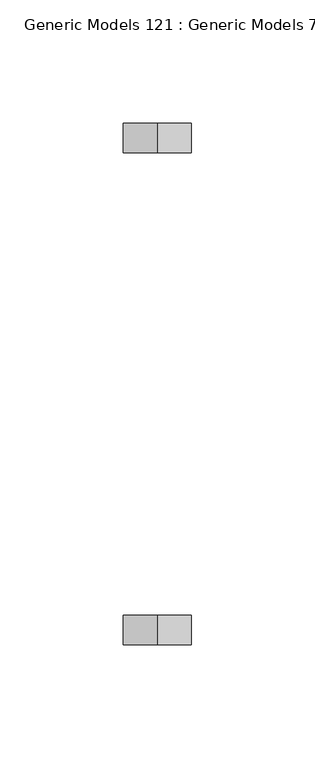
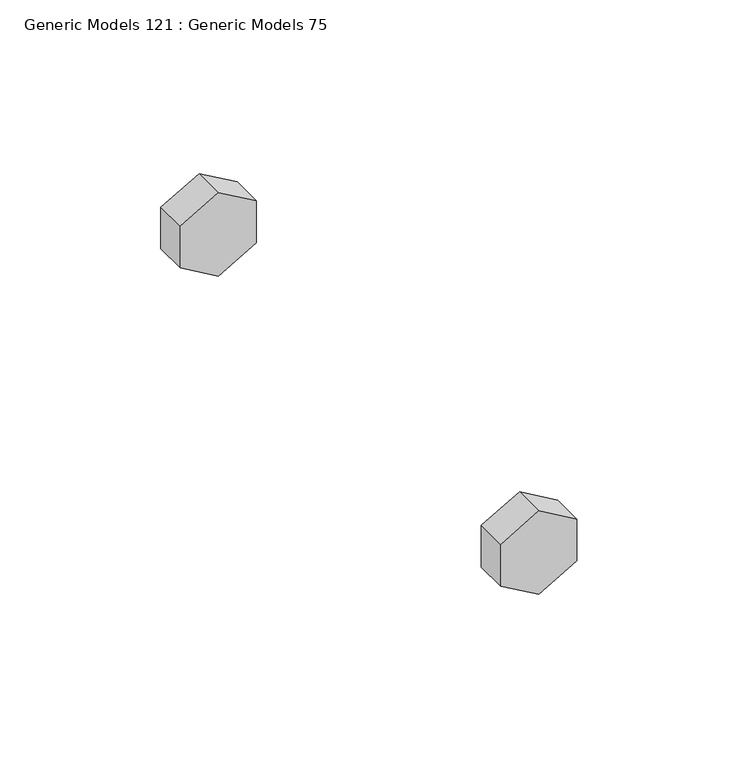
"""IFC4 building model written with IfcOpenShell, lengths in millimetres: proxy geometry, Generic Models 121 : Generic Models 75."""

from ifc_helpers import new_model, si_unit, frame, origin, place, context, project, spatial, polyline, outline, extrude, source, transform, mapped, element, save


def generic_models_121_generic_models_75_dd651f87(model_context):
    return source(origin(), model_context, "Body", "SweptSolid", [
        extrude(outline(polyline([(268993.7462802, 31974.4067029), (268977.9097067, 31974.4067029), (268969.99142, 31988.1215778), (268977.9097067, 32001.8364528), (268993.7462802, 32001.8364528), (269001.664567, 31988.1215778), (268993.7462802, 31974.4067029)])), frame((0.0, 36501.0832942, 0.0), z_axis=(0.0, 1.0, 0.0), x_axis=(0.0, 0.0, 1.0)), (0.0, 0.0, 1.0), 11.90625),
        extrude(outline(polyline([(268993.7462802, 31974.4067029), (268977.9097067, 31974.4067029), (268969.99142, 31988.1215778), (268977.9097067, 32001.8364528), (268993.7462802, 32001.8364528), (269001.664567, 31988.1215778), (268993.7462802, 31974.4067029)])), frame((0.0, 36301.8520442, 0.0), z_axis=(0.0, 1.0, 0.0), x_axis=(0.0, 0.0, 1.0)), (0.0, 0.0, 1.0), 11.90625),
    ])


if __name__ == "__main__":
    model = new_model("IFC4")
    model_context = context("Model", 3, world=origin())
    ifc_project = project(units=[si_unit("LENGTHUNIT", "METRE", prefix="MILLI")], contexts=[model_context])
    site = spatial("IfcSite", under=ifc_project)
    building = spatial("IfcBuilding", under=site)
    placement = place(None, origin())
    generic_models_121_generic_models_75_shape = generic_models_121_generic_models_75_dd651f87(model_context)
    element("IfcBuildingElementProxy", 1, Name="Generic Models 121 : Generic Models 75", ObjectType="Generic Models 121 : Generic Models 75", at=placement, inside=building, context=model_context, shape_type="MappedRepresentation", body=[
        mapped(generic_models_121_generic_models_75_shape, transform((0.0, 0.0, 0.0), x_axis=(1.0, 0.0, 0.0), y_axis=(0.0, 1.0, 0.0), z_axis=(0.0, 0.0, 1.0))),
    ])
    save(model, "model.ifc")

# Revit data of these elements
# Element 1 (IfcBuildingElementProxy, "Generic Models 121 : Generic Models 75")
#   Materials on its faces: "3/4\" GALV. THRU BOLTS"
# Materials
#   "3/4\" GALV. THRU BOLTS": class "Generic", colour RGB 105 69 171, transparency 0, Cost = 0
